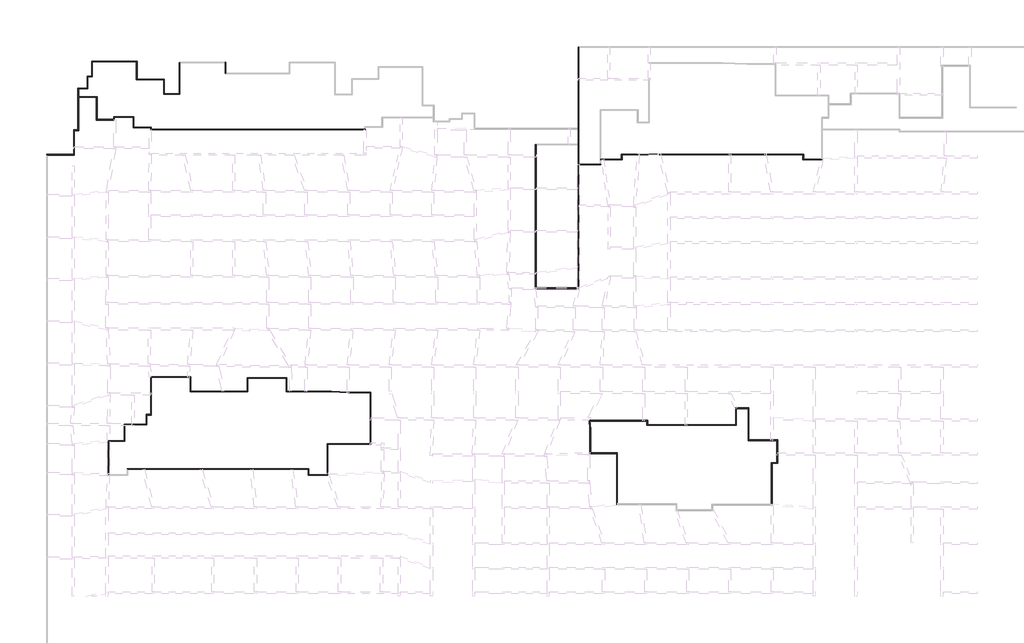
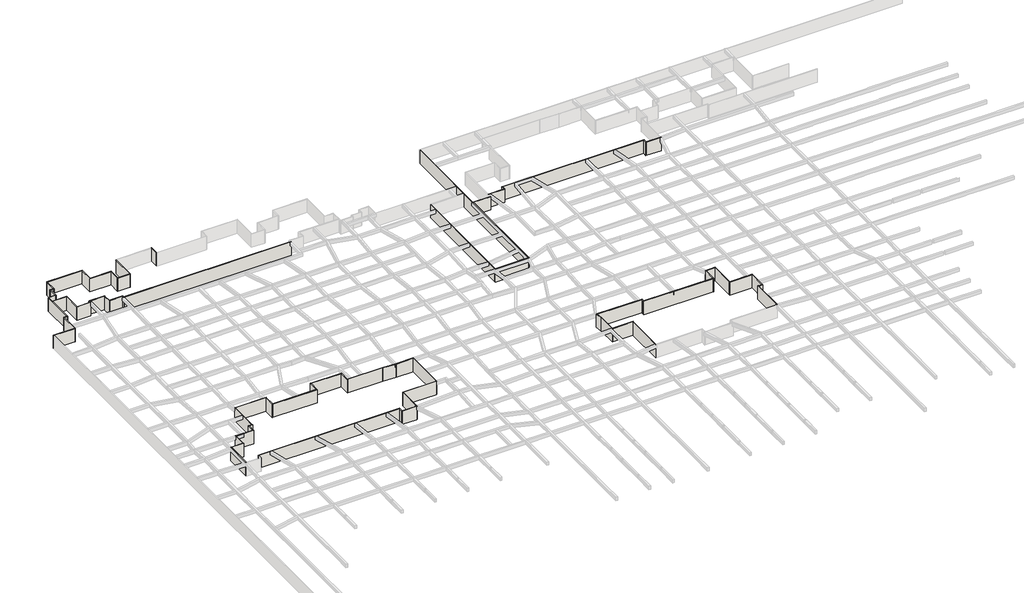
# One storey, part 7 of 45: 69 walls.
"""IFC4 building model written with IfcOpenShell, lengths in millimetres."""

from ifc_helpers import new_model, si_unit, origin, origin_with_axes, place, context, project, spatial, polyline, outline, extrude, faceted_brep, element, save

model = new_model("IFC4")

# Units and contexts
model_context = context("Model", 3, world=origin())
ifc_project = project(units=[si_unit("LENGTHUNIT", "METRE", prefix="MILLI")], contexts=[model_context])

# Site, building, storey
site = spatial("IfcSite", under=ifc_project)
building = spatial("IfcBuilding", under=site)
storey = spatial("IfcBuildingStorey", under=building, Name="户型图", Elevation=0.0)

# Walls
placement = place(None, origin())
element("IfcWall", 1, ObjectType="所有墙体", at=placement, inside=storey, context=model_context, shape_type="Brep", body=[
    faceted_brep([(-138380.5216564, 208531.9876735, 0.0), (-146800.5216564, 208531.9876735, 0.0), (-146800.5216564, 208531.9876735, 3300.0), (-138380.5216564, 208531.9876735, 3300.0), (-138380.5216564, 208411.9876735, 0.0), (-138380.5216564, 208411.9876735, 3300.0), (-138500.5216564, 208411.9876735, 3300.0), (-146680.5216564, 208411.9876735, 3300.0), (-146800.5216564, 208411.9876735, 3300.0), (-146800.5216564, 208411.9876735, 0.0), (-146680.5216564, 208411.9876735, 0.0), (-138500.5216564, 208411.9876735, 0.0)], [[[0, 1, 2, 3]], [[4, 5, 6, 7, 8, 9, 10, 11]], [[1, 0, 4, 11, 10, 9]], [[3, 2, 8, 7, 6, 5]], [[2, 1, 9, 8]], [[0, 3, 5, 4]]]),
])
element("IfcWall", 2, ObjectType="所有墙体", at=placement, inside=storey, context=model_context, shape_type="Brep", body=[
    faceted_brep([(-146800.5216564, 208411.9876735, 0.0), (-146800.5216564, 205731.9876735, 0.0), (-146800.5216564, 205611.9876735, 0.0), (-146800.5216564, 205611.9876735, 3300.0), (-146800.5216564, 205731.9876735, 3300.0), (-146800.5216564, 208411.9876735, 3300.0), (-146680.5216564, 208411.9876735, 0.0), (-146680.5216564, 208411.9876735, 3300.0), (-146680.5216564, 205611.9876735, 3300.0), (-146680.5216564, 205611.9876735, 0.0)], [[[0, 1, 2, 3, 4, 5]], [[6, 7, 8, 9]], [[2, 1, 0, 6, 9]], [[5, 4, 3, 8, 7]], [[0, 5, 7, 6]], [[3, 2, 9, 8]]]),
])
element("IfcWall", 3, ObjectType="所有墙体", at=placement, inside=storey, context=model_context, shape_type="Brep", body=[
    faceted_brep([(-146800.5216564, 205731.9876735, 0.0), (-147600.5216564, 205731.9876735, 0.0), (-147600.5216564, 205731.9876735, 3300.0), (-146800.5216564, 205731.9876735, 3300.0), (-146800.5216564, 205611.9876735, 0.0), (-146800.5216564, 205611.9876735, 3300.0), (-147480.5216564, 205611.9876735, 3300.0), (-147600.5216564, 205611.9876735, 3300.0), (-147600.5216564, 205611.9876735, 0.0), (-147480.5216564, 205611.9876735, 0.0)], [[[0, 1, 2, 3]], [[4, 5, 6, 7, 8, 9]], [[1, 0, 4, 9, 8]], [[3, 2, 7, 6, 5]], [[0, 3, 5, 4]], [[2, 1, 8, 7]]]),
])
element("IfcWall", 4, ObjectType="所有墙体", at=placement, inside=storey, context=model_context, shape_type="Brep", body=[
    faceted_brep([(-147600.5216564, 205611.9876735, 0.0), (-147600.5216564, 203531.9876735, 0.0), (-147600.5216564, 203411.9876735, 0.0), (-147600.5216564, 203411.9876735, 3300.0), (-147600.5216564, 203531.9876735, 3300.0), (-147600.5216564, 205611.9876735, 3300.0), (-147480.5216564, 205611.9876735, 0.0), (-147480.5216564, 205611.9876735, 3300.0), (-147480.5216564, 203411.9876735, 3300.0), (-147480.5216564, 203411.9876735, 0.0)], [[[0, 1, 2, 3, 4, 5]], [[6, 7, 8, 9]], [[2, 1, 0, 6, 9]], [[5, 4, 3, 8, 7]], [[0, 5, 7, 6]], [[3, 2, 9, 8]]]),
])
element("IfcWall", 5, ObjectType="所有墙体", at=placement, inside=storey, context=model_context, shape_type="Brep", body=[
    faceted_brep([(-147600.5216564, 203531.9876735, 0.0), (-149300.5216564, 203531.9876735, 0.0), (-149300.5216564, 203531.9876735, 3300.0), (-147600.5216564, 203531.9876735, 3300.0), (-147600.5216564, 203411.9876735, 0.0), (-147600.5216564, 203411.9876735, 3300.0), (-149180.5216564, 203411.9876735, 3300.0), (-149300.5216564, 203411.9876735, 3300.0), (-149300.5216564, 203411.9876735, 0.0), (-149180.5216564, 203411.9876735, 0.0)], [[[0, 1, 2, 3]], [[4, 5, 6, 7, 8, 9]], [[1, 0, 4, 9, 8]], [[3, 2, 7, 6, 5]], [[0, 3, 5, 4]], [[2, 1, 8, 7]]]),
])
element("IfcWall", 6, ObjectType="所有墙体", at=placement, inside=storey, context=model_context, shape_type="Brep", body=[
    faceted_brep([(-149300.5216564, 203411.9876735, 0.0), (-149300.5216564, 195831.9876735, 0.0), (-149300.5216564, 195711.9876735, 0.0), (-149300.5216564, 195711.9876735, 3300.0), (-149300.5216564, 195831.9876735, 3300.0), (-149300.5216564, 203411.9876735, 3300.0), (-149180.5216564, 203411.9876735, 0.0), (-149180.5216564, 203411.9876735, 3300.0), (-149180.5216564, 201971.9876735, 3300.0), (-149180.5216564, 201851.9876735, 3300.0), (-149180.5216564, 195711.9876735, 3300.0), (-149180.5216564, 195711.9876735, 0.0), (-149180.5216564, 201851.9876735, 0.0), (-149180.5216564, 201971.9876735, 0.0)], [[[0, 1, 2, 3, 4, 5]], [[6, 7, 8, 9, 10, 11, 12, 13]], [[2, 1, 0, 6, 13, 12, 11]], [[5, 4, 3, 10, 9, 8, 7]], [[0, 5, 7, 6]], [[3, 2, 11, 10]]]),
])
element("IfcWall", 7, ObjectType="所有墙体", at=placement, inside=storey, context=model_context, shape_type="Brep", body=[
    faceted_brep([(-149300.5216564, 195831.9876735, 0.0), (-150100.5216564, 195831.9876735, 0.0), (-150100.5216564, 195831.9876735, 3300.0), (-149300.5216564, 195831.9876735, 3300.0), (-149300.5216564, 195711.9876735, 0.0), (-149300.5216564, 195711.9876735, 3300.0), (-149980.5216564, 195711.9876735, 3300.0), (-150100.5216564, 195711.9876735, 3300.0), (-150100.5216564, 195711.9876735, 0.0), (-149980.5216564, 195711.9876735, 0.0)], [[[0, 1, 2, 3]], [[4, 5, 6, 7, 8, 9]], [[1, 0, 4, 9, 8]], [[3, 2, 7, 6, 5]], [[0, 3, 5, 4]], [[2, 1, 8, 7]]]),
])
element("IfcWall", 8, ObjectType="所有墙体", at=placement, inside=storey, context=model_context, shape_type="Brep", body=[
    faceted_brep([(-150100.5216564, 195711.9876735, 0.0), (-150100.5216564, 191331.9876735, 0.0), (-150100.5216564, 191211.9876735, 0.0), (-150100.5216564, 191211.9876735, 3300.0), (-150100.5216564, 191331.9876735, 3300.0), (-150100.5216564, 195711.9876735, 3300.0), (-149980.5216564, 195711.9876735, 0.0), (-149980.5216564, 195711.9876735, 3300.0), (-149980.5216564, 191211.9876735, 3300.0), (-149980.5216564, 191211.9876735, 0.0)], [[[0, 1, 2, 3, 4, 5]], [[6, 7, 8, 9]], [[2, 1, 0, 6, 9]], [[5, 4, 3, 8, 7]], [[0, 5, 7, 6]], [[3, 2, 9, 8]]]),
])
element("IfcWall", 9, ObjectType="所有墙体", at=placement, inside=storey, context=model_context, shape_type="Brep", body=[
    faceted_brep([(-150100.5216564, 191331.9876735, 0.0), (-155100.5216564, 191331.9876735, 0.0), (-155100.5216564, 191331.9876735, 3300.0), (-150100.5216564, 191331.9876735, 3300.0), (-150100.5216564, 191211.9876735, 0.0), (-150100.5216564, 191211.9876735, 3300.0), (-154980.5216564, 191211.9876735, 3300.0), (-155100.5216564, 191211.9876735, 3300.0), (-155100.5216564, 191211.9876735, 0.0), (-154980.5216564, 191211.9876735, 0.0)], [[[0, 1, 2, 3]], [[4, 5, 6, 7, 8, 9]], [[1, 0, 4, 9, 8]], [[3, 2, 7, 6, 5]], [[0, 3, 5, 4]], [[2, 1, 8, 7]]]),
])
element("IfcWall", 10, ObjectType="所有墙体", at=placement, inside=storey, context=model_context, shape_type="Brep", body=[
    faceted_brep([(-121980.5216564, 206331.9876735, 0.0), (-121980.5216564, 208331.9876735, 0.0), (-121980.5216564, 208331.9876735, 3300.0), (-121980.5216564, 206331.9876735, 3300.0), (-122100.5216564, 206331.9876735, 0.0), (-122100.5216564, 206331.9876735, 3300.0), (-122100.5216564, 208211.9876735, 3300.0), (-122100.5216564, 208331.9876735, 3300.0), (-122100.5216564, 208331.9876735, 0.0), (-122100.5216564, 208211.9876735, 0.0)], [[[0, 1, 2, 3]], [[4, 5, 6, 7, 8, 9]], [[1, 0, 4, 9, 8]], [[3, 2, 7, 6, 5]], [[0, 3, 5, 4]], [[2, 1, 8, 7]]]),
])
element("IfcWall", 11, ObjectType="所有墙体", at=placement, inside=storey, context=model_context, shape_type="Brep", body=[
    faceted_brep([(-130600.5216564, 208211.9876735, 0.0), (-130600.5216564, 202531.9876735, 0.0), (-130600.5216564, 202411.9876735, 0.0), (-130600.5216564, 202411.9876735, 3300.0), (-130600.5216564, 202531.9876735, 3300.0), (-130600.5216564, 208211.9876735, 3300.0), (-130480.5216564, 208211.9876735, 0.0), (-130480.5216564, 208211.9876735, 3300.0), (-130480.5216564, 202411.9876735, 3300.0), (-130480.5216564, 202411.9876735, 0.0)], [[[0, 1, 2, 3, 4, 5]], [[6, 7, 8, 9]], [[2, 1, 0, 6, 9]], [[5, 4, 3, 8, 7]], [[0, 5, 7, 6]], [[3, 2, 9, 8]]]),
])
element("IfcWall", 12, ObjectType="所有墙体", at=placement, inside=storey, context=model_context, shape_type="Brep", body=[
    faceted_brep([(-130600.5216564, 202531.9876735, 0.0), (-133380.5216564, 202531.9876735, 0.0), (-133500.5216564, 202531.9876735, 0.0), (-133500.5216564, 202531.9876735, 3300.0), (-133380.5216564, 202531.9876735, 3300.0), (-130600.5216564, 202531.9876735, 3300.0), (-130600.5216564, 202411.9876735, 0.0), (-130600.5216564, 202411.9876735, 3300.0), (-133500.5216564, 202411.9876735, 3300.0), (-133500.5216564, 202411.9876735, 0.0)], [[[0, 1, 2, 3, 4, 5]], [[6, 7, 8, 9]], [[2, 1, 0, 6, 9]], [[5, 4, 3, 8, 7]], [[0, 5, 7, 6]], [[3, 2, 9, 8]]]),
])
element("IfcWall", 13, ObjectType="所有墙体", at=placement, inside=storey, context=model_context, shape_type="Brep", body=[
    faceted_brep([(-133380.5216564, 202531.9876735, 0.0), (-133380.5216564, 205231.9876735, 0.0), (-133380.5216564, 205231.9876735, 3300.0), (-133380.5216564, 202531.9876735, 3300.0), (-133500.5216564, 202531.9876735, 0.0), (-133500.5216564, 202531.9876735, 3300.0), (-133500.5216564, 205111.9876735, 3300.0), (-133500.5216564, 205231.9876735, 3300.0), (-133500.5216564, 205231.9876735, 0.0), (-133500.5216564, 205111.9876735, 0.0)], [[[0, 1, 2, 3]], [[4, 5, 6, 7, 8, 9]], [[1, 0, 4, 9, 8]], [[3, 2, 7, 6, 5]], [[0, 3, 5, 4]], [[2, 1, 8, 7]]]),
])
element("IfcWall", 14, ObjectType="所有墙体", at=placement, inside=storey, context=model_context, shape_type="Brep", body=[
    faceted_brep([(-133500.5216564, 205231.9876735, 0.0), (-138380.5216564, 205231.9876735, 0.0), (-138500.5216564, 205231.9876735, 0.0), (-138500.5216564, 205231.9876735, 3300.0), (-138380.5216564, 205231.9876735, 3300.0), (-133500.5216564, 205231.9876735, 3300.0), (-133500.5216564, 205111.9876735, 0.0), (-133500.5216564, 205111.9876735, 3300.0), (-138500.5216564, 205111.9876735, 3300.0), (-138500.5216564, 205111.9876735, 0.0)], [[[0, 1, 2, 3, 4, 5]], [[6, 7, 8, 9]], [[2, 1, 0, 6, 9]], [[5, 4, 3, 8, 7]], [[0, 5, 7, 6]], [[3, 2, 9, 8]]]),
])
element("IfcWall", 15, ObjectType="所有墙体", at=placement, inside=storey, context=model_context, shape_type="SweptSolid", body=[
    extrude(outline(polyline([(-138380.5216564, 208411.9876735), (-138380.5216564, 205231.9876735), (-138500.5216564, 205231.9876735), (-138500.5216564, 208411.9876735), (-138380.5216564, 208411.9876735)])), origin_with_axes(), (0.0, 0.0, 1.0), 3300.0),
])
element("IfcWall", 16, ObjectType="所有墙体", at=placement, inside=storey, context=model_context, shape_type="Brep", body=[
    faceted_brep([(-149180.5216564, 201851.9876735, 0.0), (-145900.5216564, 201851.9876735, 0.0), (-145780.5216564, 201851.9876735, 0.0), (-145780.5216564, 201851.9876735, 3300.0), (-145900.5216564, 201851.9876735, 3300.0), (-149180.5216564, 201851.9876735, 3300.0), (-149180.5216564, 201971.9876735, 0.0), (-149180.5216564, 201971.9876735, 3300.0), (-145780.5216564, 201971.9876735, 3300.0), (-145780.5216564, 201971.9876735, 0.0)], [[[0, 1, 2, 3, 4, 5]], [[6, 7, 8, 9]], [[2, 1, 0, 6, 9]], [[5, 4, 3, 8, 7]], [[0, 5, 7, 6]], [[3, 2, 9, 8]]]),
])
element("IfcWall", 17, ObjectType="所有墙体", at=placement, inside=storey, context=model_context, shape_type="Brep", body=[
    faceted_brep([(-145900.5216564, 201851.9876735, 0.0), (-145900.5216564, 197651.9876735, 0.0), (-145900.5216564, 197651.9876735, 3300.0), (-145900.5216564, 201851.9876735, 3300.0), (-145780.5216564, 201851.9876735, 0.0), (-145780.5216564, 201851.9876735, 3300.0), (-145780.5216564, 197771.9876735, 3300.0), (-145780.5216564, 197651.9876735, 3300.0), (-145780.5216564, 197651.9876735, 0.0), (-145780.5216564, 197771.9876735, 0.0)], [[[0, 1, 2, 3]], [[4, 5, 6, 7, 8, 9]], [[1, 0, 4, 9, 8]], [[3, 2, 7, 6, 5]], [[0, 3, 5, 4]], [[2, 1, 8, 7]]]),
])
element("IfcWall", 18, ObjectType="所有墙体", at=placement, inside=storey, context=model_context, shape_type="Brep", body=[
    faceted_brep([(-145780.5216564, 197651.9876735, 0.0), (-142580.5216564, 197651.9876735, 0.0), (-142580.5216564, 197651.9876735, 3300.0), (-145780.5216564, 197651.9876735, 3300.0), (-145780.5216564, 197771.9876735, 0.0), (-145780.5216564, 197771.9876735, 3300.0), (-142700.5216564, 197771.9876735, 3300.0), (-142580.5216564, 197771.9876735, 3300.0), (-142580.5216564, 197771.9876735, 0.0), (-142700.5216564, 197771.9876735, 0.0)], [[[0, 1, 2, 3]], [[4, 5, 6, 7, 8, 9]], [[1, 0, 4, 9, 8]], [[3, 2, 7, 6, 5]], [[0, 3, 5, 4]], [[2, 1, 8, 7]]]),
])
element("IfcWall", 19, ObjectType="所有墙体", at=placement, inside=storey, context=model_context, shape_type="Brep", body=[
    faceted_brep([(-142580.5216564, 197771.9876735, 0.0), (-142580.5216564, 198151.9876735, 0.0), (-142580.5216564, 198271.9876735, 0.0), (-142580.5216564, 198271.9876735, 3300.0), (-142580.5216564, 198151.9876735, 3300.0), (-142580.5216564, 197771.9876735, 3300.0), (-142700.5216564, 197771.9876735, 0.0), (-142700.5216564, 197771.9876735, 3300.0), (-142700.5216564, 198271.9876735, 3300.0), (-142700.5216564, 198271.9876735, 0.0)], [[[0, 1, 2, 3, 4, 5]], [[6, 7, 8, 9]], [[2, 1, 0, 6, 9]], [[5, 4, 3, 8, 7]], [[0, 5, 7, 6]], [[3, 2, 9, 8]]]),
])
element("IfcWall", 20, ObjectType="所有墙体", at=placement, inside=storey, context=model_context, shape_type="Brep", body=[
    faceted_brep([(-142580.5216564, 198151.9876735, 0.0), (-139100.5216564, 198151.9876735, 0.0), (-138980.5216564, 198151.9876735, 0.0), (-138980.5216564, 198151.9876735, 3300.0), (-139100.5216564, 198151.9876735, 3300.0), (-142580.5216564, 198151.9876735, 3300.0), (-142580.5216564, 198271.9876735, 0.0), (-142580.5216564, 198271.9876735, 3300.0), (-138980.5216564, 198271.9876735, 3300.0), (-138980.5216564, 198271.9876735, 0.0)], [[[0, 1, 2, 3, 4, 5]], [[6, 7, 8, 9]], [[2, 1, 0, 6, 9]], [[5, 4, 3, 8, 7]], [[0, 5, 7, 6]], [[3, 2, 9, 8]]]),
])
element("IfcWall", 21, ObjectType="所有墙体", at=placement, inside=storey, context=model_context, shape_type="Brep", body=[
    faceted_brep([(-139100.5216564, 198151.9876735, 0.0), (-139100.5216564, 196251.9876735, 0.0), (-139100.5216564, 196251.9876735, 3300.0), (-139100.5216564, 198151.9876735, 3300.0), (-138980.5216564, 198151.9876735, 0.0), (-138980.5216564, 198151.9876735, 3300.0), (-138980.5216564, 196371.9876735, 3300.0), (-138980.5216564, 196251.9876735, 3300.0), (-138980.5216564, 196251.9876735, 0.0), (-138980.5216564, 196371.9876735, 0.0)], [[[0, 1, 2, 3]], [[4, 5, 6, 7, 8, 9]], [[1, 0, 4, 9, 8]], [[3, 2, 7, 6, 5]], [[0, 3, 5, 4]], [[2, 1, 8, 7]]]),
])
element("IfcWall", 22, ObjectType="所有墙体", at=placement, inside=storey, context=model_context, shape_type="Brep", body=[
    faceted_brep([(-138980.5216564, 196251.9876735, 0.0), (-135900.5216564, 196251.9876735, 0.0), (-135780.5216564, 196251.9876735, 0.0), (-135780.5216564, 196251.9876735, 3300.0), (-135900.5216564, 196251.9876735, 3300.0), (-138980.5216564, 196251.9876735, 3300.0), (-138980.5216564, 196371.9876735, 0.0), (-138980.5216564, 196371.9876735, 3300.0), (-135780.5216564, 196371.9876735, 3300.0), (-135780.5216564, 196371.9876735, 0.0)], [[[0, 1, 2, 3, 4, 5]], [[6, 7, 8, 9]], [[2, 1, 0, 6, 9]], [[5, 4, 3, 8, 7]], [[0, 5, 7, 6]], [[3, 2, 9, 8]]]),
])
element("IfcWall", 23, ObjectType="所有墙体", at=placement, inside=storey, context=model_context, shape_type="Brep", body=[
    faceted_brep([(-135900.5216564, 196251.9876735, 0.0), (-135900.5216564, 195851.9876735, 0.0), (-135900.5216564, 195851.9876735, 3300.0), (-135900.5216564, 196251.9876735, 3300.0), (-135780.5216564, 196251.9876735, 0.0), (-135780.5216564, 196251.9876735, 3300.0), (-135780.5216564, 195971.9876735, 3300.0), (-135780.5216564, 195851.9876735, 3300.0), (-135780.5216564, 195851.9876735, 0.0), (-135780.5216564, 195971.9876735, 0.0)], [[[0, 1, 2, 3]], [[4, 5, 6, 7, 8, 9]], [[1, 0, 4, 9, 8]], [[3, 2, 7, 6, 5]], [[0, 3, 5, 4]], [[2, 1, 8, 7]]]),
])
element("IfcWall", 24, ObjectType="所有墙体", at=placement, inside=storey, context=model_context, shape_type="Brep", body=[
    faceted_brep([(-135780.5216564, 195851.9876735, 0.0), (-96280.5216564, 195851.9876735, 0.0), (-96280.5216564, 195851.9876735, 3300.0), (-135780.5216564, 195851.9876735, 3300.0), (-135780.5216564, 195971.9876735, 0.0), (-135780.5216564, 195971.9876735, 3300.0), (-96400.5216564, 195971.9876735, 3300.0), (-96280.5216564, 195971.9876735, 3300.0), (-96280.5216564, 195971.9876735, 0.0), (-96400.5216564, 195971.9876735, 0.0)], [[[0, 1, 2, 3]], [[4, 5, 6, 7, 8, 9]], [[1, 0, 4, 9, 8]], [[3, 2, 7, 6, 5]], [[0, 3, 5, 4]], [[2, 1, 8, 7]]]),
])
element("IfcWall", 25, ObjectType="所有墙体", at=placement, inside=storey, context=model_context, shape_type="Brep", body=[
    faceted_brep([(-57000.5216564, 211111.9876735, 0.0), (-57000.5216564, 196131.9876735, 0.0), (-57000.5216564, 196011.9876735, 0.0), (-57000.5216564, 193202.3986126, 0.0), (-57000.5216564, 193082.3986126, 0.0), (-57000.5216564, 166676.8884871, 0.0), (-57000.5216564, 166556.8884871, 0.0), (-57000.5216564, 166556.8884871, 3300.0), (-57000.5216564, 166676.8884871, 3300.0), (-57000.5216564, 193082.3986126, 3300.0), (-57000.5216564, 193202.3986126, 3300.0), (-57000.5216564, 196011.9876735, 3300.0), (-57000.5216564, 196131.9876735, 3300.0), (-57000.5216564, 211111.9876735, 3300.0), (-56880.5216564, 211111.9876735, 0.0), (-56880.5216564, 211111.9876735, 3300.0), (-56880.5216564, 189542.3986126, 3300.0), (-56880.5216564, 189422.3986126, 3300.0), (-56880.5216564, 166556.8884871, 3300.0), (-56880.5216564, 166556.8884871, 0.0), (-56880.5216564, 189422.3986126, 0.0), (-56880.5216564, 189542.3986126, 0.0)], [[[0, 1, 2, 3, 4, 5, 6, 7, 8, 9, 10, 11, 12, 13]], [[14, 15, 16, 17, 18, 19, 20, 21]], [[6, 5, 4, 3, 2, 1, 0, 14, 21, 20, 19]], [[13, 12, 11, 10, 9, 8, 7, 18, 17, 16, 15]], [[7, 6, 19, 18]], [[0, 13, 15, 14]]]),
])
element("IfcWall", 26, ObjectType="所有墙体", at=placement, inside=storey, context=model_context, shape_type="Brep", body=[
    faceted_brep([(-57000.5216564, 166676.8884871, 0.0), (-64742.224124, 166676.8884871, 0.0), (-64862.224124, 166676.8884871, 0.0), (-64862.224124, 166676.8884871, 3300.0), (-64742.224124, 166676.8884871, 3300.0), (-57000.5216564, 166676.8884871, 3300.0), (-57000.5216564, 166556.8884871, 0.0), (-57000.5216564, 166556.8884871, 3300.0), (-64862.224124, 166556.8884871, 3300.0), (-64862.224124, 166556.8884871, 0.0)], [[[0, 1, 2, 3, 4, 5]], [[6, 7, 8, 9]], [[2, 1, 0, 6, 9]], [[5, 4, 3, 8, 7]], [[0, 5, 7, 6]], [[3, 2, 9, 8]]]),
])
element("IfcWall", 27, ObjectType="所有墙体", at=placement, inside=storey, context=model_context, shape_type="SweptSolid", body=[
    extrude(outline(polyline([(-64742.224124, 193082.3986126), (-64742.224124, 166676.8884871), (-64862.224124, 166676.8884871), (-64862.224124, 193082.3986126), (-64742.224124, 193082.3986126)])), origin_with_axes(), (0.0, 0.0, 1.0), 3300.0),
])
element("IfcWall", 28, ObjectType="所有墙体", at=placement, inside=storey, context=model_context, shape_type="Brep", body=[
    faceted_brep([(-56880.5216564, 189422.3986126, 0.0), (-52780.5216564, 189422.3986126, 0.0), (-52780.5216564, 189422.3986126, 3300.0), (-56880.5216564, 189422.3986126, 3300.0), (-56880.5216564, 189542.3986126, 0.0), (-56880.5216564, 189542.3986126, 3300.0), (-52900.5216564, 189542.3986126, 3300.0), (-52780.5216564, 189542.3986126, 3300.0), (-52780.5216564, 189542.3986126, 0.0), (-52900.5216564, 189542.3986126, 0.0)], [[[0, 1, 2, 3]], [[4, 5, 6, 7, 8, 9]], [[1, 0, 4, 9, 8]], [[3, 2, 7, 6, 5]], [[0, 3, 5, 4]], [[2, 1, 8, 7]]]),
])
element("IfcWall", 29, ObjectType="所有墙体", at=placement, inside=storey, context=model_context, shape_type="Brep", body=[
    faceted_brep([(-52780.5216564, 190322.3986126, 0.0), (-48880.5216564, 190322.3986126, 0.0), (-48880.5216564, 190322.3986126, 3300.0), (-52780.5216564, 190322.3986126, 3300.0), (-52780.5216564, 190442.3986126, 0.0), (-52780.5216564, 190442.3986126, 3300.0), (-49000.5216564, 190442.3986126, 3300.0), (-48880.5216564, 190442.3986126, 3300.0), (-48880.5216564, 190442.3986126, 0.0), (-49000.5216564, 190442.3986126, 0.0)], [[[0, 1, 2, 3]], [[4, 5, 6, 7, 8, 9]], [[1, 0, 4, 9, 8]], [[3, 2, 7, 6, 5]], [[0, 3, 5, 4]], [[2, 1, 8, 7]]]),
])
element("IfcWall", 30, ObjectType="所有墙体", at=placement, inside=storey, context=model_context, shape_type="Brep", body=[
    faceted_brep([(-48880.5216564, 190442.3986126, 0.0), (-48880.5216564, 191222.3986126, 0.0), (-48880.5216564, 191342.3986126, 0.0), (-48880.5216564, 191342.3986126, 3300.0), (-48880.5216564, 191222.3986126, 3300.0), (-48880.5216564, 190442.3986126, 3300.0), (-49000.5216564, 190442.3986126, 0.0), (-49000.5216564, 190442.3986126, 3300.0), (-49000.5216564, 191342.3986126, 3300.0), (-49000.5216564, 191342.3986126, 0.0)], [[[0, 1, 2, 3, 4, 5]], [[6, 7, 8, 9]], [[2, 1, 0, 6, 9]], [[5, 4, 3, 8, 7]], [[0, 5, 7, 6]], [[3, 2, 9, 8]]]),
])
element("IfcWall", 31, ObjectType="所有墙体", at=placement, inside=storey, context=model_context, shape_type="Brep", body=[
    faceted_brep([(-48880.5216564, 191222.3986126, 0.0), (-15500.5216564, 191222.3986126, 0.0), (-15380.5216564, 191222.3986126, 0.0), (-15380.5216564, 191222.3986126, 3300.0), (-15500.5216564, 191222.3986126, 3300.0), (-48880.5216564, 191222.3986126, 3300.0), (-48880.5216564, 191342.3986126, 0.0), (-48880.5216564, 191342.3986126, 3300.0), (-15380.5216564, 191342.3986126, 3300.0), (-15380.5216564, 191342.3986126, 0.0)], [[[0, 1, 2, 3, 4, 5]], [[6, 7, 8, 9]], [[2, 1, 0, 6, 9]], [[5, 4, 3, 8, 7]], [[0, 5, 7, 6]], [[3, 2, 9, 8]]]),
])
element("IfcWall", 32, ObjectType="所有墙体", at=placement, inside=storey, context=model_context, shape_type="Brep", body=[
    faceted_brep([(-15500.5216564, 191222.3986126, 0.0), (-15500.5216564, 190322.3986126, 0.0), (-15500.5216564, 190322.3986126, 3300.0), (-15500.5216564, 191222.3986126, 3300.0), (-15380.5216564, 191222.3986126, 0.0), (-15380.5216564, 191222.3986126, 3300.0), (-15380.5216564, 190442.3986126, 3300.0), (-15380.5216564, 190322.3986126, 3300.0), (-15380.5216564, 190322.3986126, 0.0), (-15380.5216564, 190442.3986126, 0.0)], [[[0, 1, 2, 3]], [[4, 5, 6, 7, 8, 9]], [[1, 0, 4, 9, 8]], [[3, 2, 7, 6, 5]], [[0, 3, 5, 4]], [[2, 1, 8, 7]]]),
])
element("IfcWall", 33, ObjectType="所有墙体", at=placement, inside=storey, context=model_context, shape_type="Brep", body=[
    faceted_brep([(-15380.5216564, 190322.3986126, 0.0), (-11926.7821096, 190322.3986126, 0.0), (-11926.7821096, 190322.3986126, 3300.0), (-15380.5216564, 190322.3986126, 3300.0), (-15380.5216564, 190442.3986126, 0.0), (-15380.5216564, 190442.3986126, 3300.0), (-12046.7821096, 190442.3986126, 3300.0), (-11926.7821096, 190442.3986126, 3300.0), (-11926.7821096, 190442.3986126, 0.0), (-12046.7821096, 190442.3986126, 0.0)], [[[0, 1, 2, 3]], [[4, 5, 6, 7, 8, 9]], [[1, 0, 4, 9, 8]], [[3, 2, 7, 6, 5]], [[0, 3, 5, 4]], [[2, 1, 8, 7]]]),
])
element("IfcWall", 34, ObjectType="所有墙体", at=placement, inside=storey, context=model_context, shape_type="Brep", body=[
    faceted_brep([(-140683.5692432, 141410.7814363, 0.0), (-136572.9151571, 141410.7814363, 0.0), (-136572.9151571, 141410.7814363, 3300.0), (-140683.5692432, 141410.7814363, 3300.0), (-140683.5692432, 141530.7814363, 0.0), (-140683.5692432, 141530.7814363, 3300.0), (-136692.9151571, 141530.7814363, 3300.0), (-136572.9151571, 141530.7814363, 3300.0), (-136572.9151571, 141530.7814363, 0.0), (-136692.9151571, 141530.7814363, 0.0)], [[[0, 1, 2, 3]], [[4, 5, 6, 7, 8, 9]], [[1, 0, 4, 9, 8]], [[3, 2, 7, 6, 5]], [[2, 1, 8, 7]], [[0, 3, 5, 4]]]),
])
element("IfcWall", 35, ObjectType="所有墙体", at=placement, inside=storey, context=model_context, shape_type="Brep", body=[
    faceted_brep([(-136572.9151571, 141530.7814363, 0.0), (-136572.9151571, 143210.7814363, 0.0), (-136572.9151571, 143330.7814363, 0.0), (-136572.9151571, 143330.7814363, 3300.0), (-136572.9151571, 143210.7814363, 3300.0), (-136572.9151571, 141530.7814363, 3300.0), (-136692.9151571, 141530.7814363, 0.0), (-136692.9151571, 141530.7814363, 3300.0), (-136692.9151571, 143330.7814363, 3300.0), (-136692.9151571, 143330.7814363, 0.0)], [[[0, 1, 2, 3, 4, 5]], [[6, 7, 8, 9]], [[2, 1, 0, 6, 9]], [[5, 4, 3, 8, 7]], [[0, 5, 7, 6]], [[3, 2, 9, 8]]]),
])
element("IfcWall", 36, ObjectType="所有墙体", at=placement, inside=storey, context=model_context, shape_type="Brep", body=[
    faceted_brep([(-136572.9151571, 143210.7814363, 0.0), (-135772.9151571, 143210.7814363, 0.0), (-135772.9151571, 143210.7814363, 3300.0), (-136572.9151571, 143210.7814363, 3300.0), (-136572.9151571, 143330.7814363, 0.0), (-136572.9151571, 143330.7814363, 3300.0), (-135892.9151571, 143330.7814363, 3300.0), (-135772.9151571, 143330.7814363, 3300.0), (-135772.9151571, 143330.7814363, 0.0), (-135892.9151571, 143330.7814363, 0.0)], [[[0, 1, 2, 3]], [[4, 5, 6, 7, 8, 9]], [[1, 0, 4, 9, 8]], [[3, 2, 7, 6, 5]], [[0, 3, 5, 4]], [[2, 1, 8, 7]]]),
])
element("IfcWall", 37, ObjectType="所有墙体", at=placement, inside=storey, context=model_context, shape_type="Brep", body=[
    faceted_brep([(-135772.9151571, 143330.7814363, 0.0), (-135772.9151571, 150210.7814363, 0.0), (-135772.9151571, 150330.7814363, 0.0), (-135772.9151571, 150330.7814363, 3300.0), (-135772.9151571, 150210.7814363, 3300.0), (-135772.9151571, 143330.7814363, 3300.0), (-135892.9151571, 143330.7814363, 0.0), (-135892.9151571, 143330.7814363, 3300.0), (-135892.9151571, 150330.7814363, 3300.0), (-135892.9151571, 150330.7814363, 0.0)], [[[0, 1, 2, 3, 4, 5]], [[6, 7, 8, 9]], [[2, 1, 0, 6, 9]], [[5, 4, 3, 8, 7]], [[0, 5, 7, 6]], [[3, 2, 9, 8]]]),
])
element("IfcWall", 38, ObjectType="所有墙体", at=placement, inside=storey, context=model_context, shape_type="Brep", body=[
    faceted_brep([(-135772.9151571, 150210.7814363, 0.0), (-128592.9151571, 150210.7814363, 0.0), (-128472.9151571, 150210.7814363, 0.0), (-128472.9151571, 150210.7814363, 3300.0), (-128592.9151571, 150210.7814363, 3300.0), (-135772.9151571, 150210.7814363, 3300.0), (-135772.9151571, 150330.7814363, 0.0), (-135772.9151571, 150330.7814363, 3300.0), (-128472.9151571, 150330.7814363, 3300.0), (-128472.9151571, 150330.7814363, 0.0)], [[[0, 1, 2, 3, 4, 5]], [[6, 7, 8, 9]], [[2, 1, 0, 6, 9]], [[5, 4, 3, 8, 7]], [[0, 5, 7, 6]], [[3, 2, 9, 8]]]),
])
element("IfcWall", 39, ObjectType="所有墙体", at=placement, inside=storey, context=model_context, shape_type="Brep", body=[
    faceted_brep([(-128592.9151571, 150210.7814363, 0.0), (-128592.9151571, 147510.7814363, 0.0), (-128592.9151571, 147510.7814363, 3300.0), (-128592.9151571, 150210.7814363, 3300.0), (-128472.9151571, 150210.7814363, 0.0), (-128472.9151571, 150210.7814363, 3300.0), (-128472.9151571, 147630.7814363, 3300.0), (-128472.9151571, 147510.7814363, 3300.0), (-128472.9151571, 147510.7814363, 0.0), (-128472.9151571, 147630.7814363, 0.0)], [[[0, 1, 2, 3]], [[4, 5, 6, 7, 8, 9]], [[1, 0, 4, 9, 8]], [[3, 2, 7, 6, 5]], [[0, 3, 5, 4]], [[2, 1, 8, 7]]]),
])
element("IfcWall", 40, ObjectType="所有墙体", at=placement, inside=storey, context=model_context, shape_type="Brep", body=[
    faceted_brep([(-128472.9151571, 147510.7814363, 0.0), (-117972.9151571, 147510.7814363, 0.0), (-117972.9151571, 147510.7814363, 3300.0), (-128472.9151571, 147510.7814363, 3300.0), (-128472.9151571, 147630.7814363, 0.0), (-128472.9151571, 147630.7814363, 3300.0), (-118092.9151571, 147630.7814363, 3300.0), (-117972.9151571, 147630.7814363, 3300.0), (-117972.9151571, 147630.7814363, 0.0), (-118092.9151571, 147630.7814363, 0.0)], [[[0, 1, 2, 3]], [[4, 5, 6, 7, 8, 9]], [[1, 0, 4, 9, 8]], [[3, 2, 7, 6, 5]], [[0, 3, 5, 4]], [[2, 1, 8, 7]]]),
])
element("IfcWall", 41, ObjectType="所有墙体", at=placement, inside=storey, context=model_context, shape_type="Brep", body=[
    faceted_brep([(-117972.9151571, 147630.7814363, 0.0), (-117972.9151571, 150010.7814363, 0.0), (-117972.9151571, 150130.7814363, 0.0), (-117972.9151571, 150130.7814363, 3300.0), (-117972.9151571, 150010.7814363, 3300.0), (-117972.9151571, 147630.7814363, 3300.0), (-118092.9151571, 147630.7814363, 0.0), (-118092.9151571, 147630.7814363, 3300.0), (-118092.9151571, 150130.7814363, 3300.0), (-118092.9151571, 150130.7814363, 0.0)], [[[0, 1, 2, 3, 4, 5]], [[6, 7, 8, 9]], [[2, 1, 0, 6, 9]], [[5, 4, 3, 8, 7]], [[0, 5, 7, 6]], [[3, 2, 9, 8]]]),
])
element("IfcWall", 42, ObjectType="所有墙体", at=placement, inside=storey, context=model_context, shape_type="Brep", body=[
    faceted_brep([(-117972.9151571, 150010.7814363, 0.0), (-110892.9151571, 150010.7814363, 0.0), (-110772.9151571, 150010.7814363, 0.0), (-110772.9151571, 150010.7814363, 3300.0), (-110892.9151571, 150010.7814363, 3300.0), (-117972.9151571, 150010.7814363, 3300.0), (-117972.9151571, 150130.7814363, 0.0), (-117972.9151571, 150130.7814363, 3300.0), (-110772.9151571, 150130.7814363, 3300.0), (-110772.9151571, 150130.7814363, 0.0)], [[[0, 1, 2, 3, 4, 5]], [[6, 7, 8, 9]], [[2, 1, 0, 6, 9]], [[5, 4, 3, 8, 7]], [[0, 5, 7, 6]], [[3, 2, 9, 8]]]),
])
element("IfcWall", 43, ObjectType="所有墙体", at=placement, inside=storey, context=model_context, shape_type="Brep", body=[
    faceted_brep([(-110892.9151571, 150010.7814363, 0.0), (-110892.9151571, 147510.7814363, 0.0), (-110892.9151571, 147510.7814363, 3300.0), (-110892.9151571, 150010.7814363, 3300.0), (-110772.9151571, 150010.7814363, 0.0), (-110772.9151571, 150010.7814363, 3300.0), (-110772.9151571, 147630.7814363, 3300.0), (-110772.9151571, 147510.7814363, 3300.0), (-110772.9151571, 147510.7814363, 0.0), (-110772.9151571, 147630.7814363, 0.0)], [[[0, 1, 2, 3]], [[4, 5, 6, 7, 8, 9]], [[1, 0, 4, 9, 8]], [[3, 2, 7, 6, 5]], [[0, 3, 5, 4]], [[2, 1, 8, 7]]]),
])
element("IfcWall", 44, ObjectType="所有墙体", at=placement, inside=storey, context=model_context, shape_type="SweptSolid", body=[
    extrude(outline(polyline([(-102534.7708159, 147510.7814363), (-110772.9151571, 147510.7814363), (-110772.9151571, 147630.7814363), (-102531.0594982, 147630.7814363), (-102534.7708159, 147510.7814363)])), origin_with_axes(), (0.0, 0.0, 1.0), 3300.0),
])
element("IfcWall", 45, ObjectType="所有墙体", at=placement, inside=storey, context=model_context, shape_type="SweptSolid", body=[
    extrude(outline(polyline([(-99445.424902, 147319.5060773), (-102534.7708159, 147510.7814363), (-102531.0594982, 147630.7814363), (-99441.7135844, 147439.5060773), (-99445.424902, 147319.5060773)])), origin_with_axes(), (0.0, 0.0, 1.0), 3300.0),
])
element("IfcWall", 46, ObjectType="所有墙体", at=placement, inside=storey, context=model_context, shape_type="Brep", body=[
    faceted_brep([(-99445.424902, 147319.5060773, 0.0), (-95403.5692432, 147319.5060773, 0.0), (-95283.5692432, 147319.5060773, 0.0), (-95283.5692432, 147319.5060773, 3300.0), (-95403.5692432, 147319.5060773, 3300.0), (-99445.424902, 147319.5060773, 3300.0), (-99441.7135844, 147439.5060773, 0.0), (-99441.7135844, 147439.5060773, 3300.0), (-95283.5692432, 147439.5060773, 3300.0), (-95283.5692432, 147439.5060773, 0.0)], [[[0, 1, 2, 3, 4, 5]], [[6, 7, 8, 9]], [[2, 1, 0, 6, 9]], [[5, 4, 3, 8, 7]], [[0, 5, 7, 6]], [[3, 2, 9, 8]]]),
])
element("IfcWall", 47, ObjectType="所有墙体", at=placement, inside=storey, context=model_context, shape_type="Brep", body=[
    faceted_brep([(-95403.5692432, 147319.5060773, 0.0), (-95403.5692432, 137939.5060773, 0.0), (-95403.5692432, 137819.5060773, 0.0), (-95403.5692432, 137819.5060773, 3300.0), (-95403.5692432, 137939.5060773, 3300.0), (-95403.5692432, 147319.5060773, 3300.0), (-95283.5692432, 147319.5060773, 0.0), (-95283.5692432, 147319.5060773, 3300.0), (-95283.5692432, 137819.5060773, 3300.0), (-95283.5692432, 137819.5060773, 0.0)], [[[0, 1, 2, 3, 4, 5]], [[6, 7, 8, 9]], [[2, 1, 0, 6, 9]], [[5, 4, 3, 8, 7]], [[0, 5, 7, 6]], [[3, 2, 9, 8]]]),
])
element("IfcWall", 48, ObjectType="所有墙体", at=placement, inside=storey, context=model_context, shape_type="Brep", body=[
    faceted_brep([(-95403.5692432, 137939.5060773, 0.0), (-103303.5692432, 137939.5060773, 0.0), (-103303.5692432, 137939.5060773, 3300.0), (-95403.5692432, 137939.5060773, 3300.0), (-95403.5692432, 137819.5060773, 0.0), (-95403.5692432, 137819.5060773, 3300.0), (-103183.5692432, 137819.5060773, 3300.0), (-103303.5692432, 137819.5060773, 3300.0), (-103303.5692432, 137819.5060773, 0.0), (-103183.5692432, 137819.5060773, 0.0)], [[[0, 1, 2, 3]], [[4, 5, 6, 7, 8, 9]], [[1, 0, 4, 9, 8]], [[3, 2, 7, 6, 5]], [[0, 3, 5, 4]], [[2, 1, 8, 7]]]),
])
element("IfcWall", 49, ObjectType="所有墙体", at=placement, inside=storey, context=model_context, shape_type="Brep", body=[
    faceted_brep([(-103303.5692432, 137819.5060773, 0.0), (-103303.5692432, 132195.8564831, 0.0), (-103303.5692432, 132075.8564831, 0.0), (-103303.5692432, 132075.8564831, 3300.0), (-103303.5692432, 132195.8564831, 3300.0), (-103303.5692432, 137819.5060773, 3300.0), (-103183.5692432, 137819.5060773, 0.0), (-103183.5692432, 137819.5060773, 3300.0), (-103183.5692432, 132075.8564831, 3300.0), (-103183.5692432, 132075.8564831, 0.0)], [[[0, 1, 2, 3, 4, 5]], [[6, 7, 8, 9]], [[2, 1, 0, 6, 9]], [[5, 4, 3, 8, 7]], [[0, 5, 7, 6]], [[3, 2, 9, 8]]]),
])
element("IfcWall", 50, ObjectType="所有墙体", at=placement, inside=storey, context=model_context, shape_type="Brep", body=[
    faceted_brep([(-103303.5692432, 132195.8564831, 0.0), (-106683.5692432, 132195.8564831, 0.0), (-106803.5692432, 132195.8564831, 0.0), (-106803.5692432, 132195.8564831, 3300.0), (-106683.5692432, 132195.8564831, 3300.0), (-103303.5692432, 132195.8564831, 3300.0), (-103303.5692432, 132075.8564831, 0.0), (-103303.5692432, 132075.8564831, 3300.0), (-106803.5692432, 132075.8564831, 3300.0), (-106803.5692432, 132075.8564831, 0.0)], [[[0, 1, 2, 3, 4, 5]], [[6, 7, 8, 9]], [[2, 1, 0, 6, 9]], [[5, 4, 3, 8, 7]], [[0, 5, 7, 6]], [[3, 2, 9, 8]]]),
])
element("IfcWall", 51, ObjectType="所有墙体", at=placement, inside=storey, context=model_context, shape_type="Brep", body=[
    faceted_brep([(-106683.5692432, 132195.8564831, 0.0), (-106683.5692432, 133295.8564831, 0.0), (-106683.5692432, 133295.8564831, 3300.0), (-106683.5692432, 132195.8564831, 3300.0), (-106803.5692432, 132195.8564831, 0.0), (-106803.5692432, 132195.8564831, 3300.0), (-106803.5692432, 133175.8564831, 3300.0), (-106803.5692432, 133295.8564831, 3300.0), (-106803.5692432, 133295.8564831, 0.0), (-106803.5692432, 133175.8564831, 0.0)], [[[0, 1, 2, 3]], [[4, 5, 6, 7, 8, 9]], [[1, 0, 4, 9, 8]], [[3, 2, 7, 6, 5]], [[0, 3, 5, 4]], [[2, 1, 8, 7]]]),
])
element("IfcWall", 52, ObjectType="所有墙体", at=placement, inside=storey, context=model_context, shape_type="Brep", body=[
    faceted_brep([(-106803.5692432, 133295.8564831, 0.0), (-140203.5692432, 133295.8564831, 0.0), (-140203.5692432, 133295.8564831, 3300.0), (-106803.5692432, 133295.8564831, 3300.0), (-106803.5692432, 133175.8564831, 0.0), (-106803.5692432, 133175.8564831, 3300.0), (-140083.5692432, 133175.8564831, 3300.0), (-140203.5692432, 133175.8564831, 3300.0), (-140203.5692432, 133175.8564831, 0.0), (-140083.5692432, 133175.8564831, 0.0)], [[[0, 1, 2, 3]], [[4, 5, 6, 7, 8, 9]], [[1, 0, 4, 9, 8]], [[3, 2, 7, 6, 5]], [[0, 3, 5, 4]], [[2, 1, 8, 7]]]),
])
element("IfcWall", 53, ObjectType="所有墙体", at=placement, inside=storey, context=model_context, shape_type="Brep", body=[
    faceted_brep([(-143583.5692432, 132195.8564831, 0.0), (-143583.5692432, 138375.8564831, 0.0), (-143583.5692432, 138495.8564831, 0.0), (-143583.5692432, 138495.8564831, 3300.0), (-143583.5692432, 138375.8564831, 3300.0), (-143583.5692432, 132195.8564831, 3300.0), (-143703.5692432, 132195.8564831, 0.0), (-143703.5692432, 132195.8564831, 3300.0), (-143703.5692432, 138495.8564831, 3300.0), (-143703.5692432, 138495.8564831, 0.0)], [[[0, 1, 2, 3, 4, 5]], [[6, 7, 8, 9]], [[2, 1, 0, 6, 9]], [[5, 4, 3, 8, 7]], [[0, 5, 7, 6]], [[3, 2, 9, 8]]]),
])
element("IfcWall", 54, ObjectType="所有墙体", at=placement, inside=storey, context=model_context, shape_type="Brep", body=[
    faceted_brep([(-143583.5692432, 138375.8564831, 0.0), (-140683.5692432, 138375.8564831, 0.0), (-140683.5692432, 138375.8564831, 3300.0), (-143583.5692432, 138375.8564831, 3300.0), (-143583.5692432, 138495.8564831, 0.0), (-143583.5692432, 138495.8564831, 3300.0), (-140803.5692432, 138495.8564831, 3300.0), (-140683.5692432, 138495.8564831, 3300.0), (-140683.5692432, 138495.8564831, 0.0), (-140803.5692432, 138495.8564831, 0.0)], [[[0, 1, 2, 3]], [[4, 5, 6, 7, 8, 9]], [[1, 0, 4, 9, 8]], [[3, 2, 7, 6, 5]], [[0, 3, 5, 4]], [[2, 1, 8, 7]]]),
])
element("IfcWall", 55, ObjectType="所有墙体", at=placement, inside=storey, context=model_context, shape_type="Brep", body=[
    faceted_brep([(-140683.5692432, 138495.8564831, 0.0), (-140683.5692432, 141410.7814363, 0.0), (-140683.5692432, 141530.7814363, 0.0), (-140683.5692432, 141530.7814363, 3300.0), (-140683.5692432, 141410.7814363, 3300.0), (-140683.5692432, 138495.8564831, 3300.0), (-140803.5692432, 138495.8564831, 0.0), (-140803.5692432, 138495.8564831, 3300.0), (-140803.5692432, 141530.7814363, 3300.0), (-140803.5692432, 141530.7814363, 0.0)], [[[0, 1, 2, 3, 4, 5]], [[6, 7, 8, 9]], [[2, 1, 0, 6, 9]], [[5, 4, 3, 8, 7]], [[0, 5, 7, 6]], [[3, 2, 9, 8]]]),
])
element("IfcWall", 56, ObjectType="所有墙体", at=placement, inside=storey, context=model_context, shape_type="Brep", body=[
    faceted_brep([(-54982.3711745, 142222.9605472, 0.0), (-54807.1090692, 140555.4530019, 0.0), (-54807.1090692, 140555.4530019, 3300.0), (-54982.3711745, 142222.9605472, 3300.0), (-54861.7101809, 142222.9605472, 0.0), (-54861.7101809, 142222.9605472, 3300.0), (-54849.0976727, 142102.9605472, 3300.0), (-54687.1090692, 140561.7419354, 3300.0), (-54687.1090692, 140561.7419354, 0.0), (-54849.0976727, 142102.9605472, 0.0)], [[[0, 1, 2, 3]], [[4, 5, 6, 7, 8, 9]], [[1, 0, 4, 9, 8]], [[3, 2, 7, 6, 5]], [[2, 1, 8, 7]], [[0, 3, 5, 4]]]),
])
element("IfcWall", 57, ObjectType="所有墙体", at=placement, inside=storey, context=model_context, shape_type="Brep", body=[
    faceted_brep([(-54807.1090692, 140555.4530019, 0.0), (-54807.1090692, 136098.5974686, 0.0), (-54807.1090692, 136098.5974686, 3300.0), (-54807.1090692, 140555.4530019, 3300.0), (-54687.1090692, 140561.7419354, 0.0), (-54687.1090692, 140561.7419354, 3300.0), (-54687.1090692, 136218.5974686, 3300.0), (-54687.1090692, 136098.5974686, 3300.0), (-54687.1090692, 136098.5974686, 0.0), (-54687.1090692, 136218.5974686, 0.0)], [[[0, 1, 2, 3]], [[4, 5, 6, 7, 8, 9]], [[1, 0, 4, 9, 8]], [[3, 2, 7, 6, 5]], [[0, 3, 5, 4]], [[2, 1, 8, 7]]]),
])
element("IfcWall", 58, ObjectType="所有墙体", at=placement, inside=storey, context=model_context, shape_type="Brep", body=[
    faceted_brep([(-54687.1090692, 136098.5974686, 0.0), (-49907.1090692, 136098.5974686, 0.0), (-49787.1090692, 136098.5974686, 0.0), (-49787.1090692, 136098.5974686, 3300.0), (-49907.1090692, 136098.5974686, 3300.0), (-54687.1090692, 136098.5974686, 3300.0), (-54687.1090692, 136218.5974686, 0.0), (-54687.1090692, 136218.5974686, 3300.0), (-49787.1090692, 136218.5974686, 3300.0), (-49787.1090692, 136218.5974686, 0.0)], [[[0, 1, 2, 3, 4, 5]], [[6, 7, 8, 9]], [[2, 1, 0, 6, 9]], [[5, 4, 3, 8, 7]], [[0, 5, 7, 6]], [[3, 2, 9, 8]]]),
])
element("IfcWall", 59, ObjectType="所有墙体", at=placement, inside=storey, context=model_context, shape_type="Brep", body=[
    faceted_brep([(-49907.1090692, 136098.5974686, 0.0), (-49907.1090692, 126702.9605472, 0.0), (-49907.1090692, 126702.9605472, 3300.0), (-49907.1090692, 136098.5974686, 3300.0), (-49787.1090692, 136098.5974686, 0.0), (-49787.1090692, 136098.5974686, 3300.0), (-49787.1090692, 126822.9605472, 3300.0), (-49787.1090692, 126702.9605472, 3300.0), (-49787.1090692, 126702.9605472, 0.0), (-49787.1090692, 126822.9605472, 0.0)], [[[0, 1, 2, 3]], [[4, 5, 6, 7, 8, 9]], [[1, 0, 4, 9, 8]], [[3, 2, 7, 6, 5]], [[0, 3, 5, 4]], [[2, 1, 8, 7]]]),
])
element("IfcWall", 60, ObjectType="所有墙体", at=placement, inside=storey, context=model_context, shape_type="Brep", body=[
    faceted_brep([(-21187.1090692, 126722.9605472, 0.0), (-21187.1090692, 134302.9605472, 0.0), (-21187.1090692, 134422.9605472, 0.0), (-21187.1090692, 134422.9605472, 3300.0), (-21187.1090692, 134302.9605472, 3300.0), (-21187.1090692, 126722.9605472, 3300.0), (-21307.1090692, 126722.9605472, 0.0), (-21307.1090692, 126722.9605472, 3300.0), (-21307.1090692, 134422.9605472, 3300.0), (-21307.1090692, 134422.9605472, 0.0)], [[[0, 1, 2, 3, 4, 5]], [[6, 7, 8, 9]], [[2, 1, 0, 6, 9]], [[5, 4, 3, 8, 7]], [[0, 5, 7, 6]], [[3, 2, 9, 8]]]),
])
element("IfcWall", 61, ObjectType="所有墙体", at=placement, inside=storey, context=model_context, shape_type="Brep", body=[
    faceted_brep([(-21187.1090692, 134302.9605472, 0.0), (-20187.1090692, 134302.9605472, 0.0), (-20187.1090692, 134302.9605472, 3300.0), (-21187.1090692, 134302.9605472, 3300.0), (-21187.1090692, 134422.9605472, 0.0), (-21187.1090692, 134422.9605472, 3300.0), (-20307.1090692, 134422.9605472, 3300.0), (-20187.1090692, 134422.9605472, 3300.0), (-20187.1090692, 134422.9605472, 0.0), (-20307.1090692, 134422.9605472, 0.0)], [[[0, 1, 2, 3]], [[4, 5, 6, 7, 8, 9]], [[1, 0, 4, 9, 8]], [[3, 2, 7, 6, 5]], [[0, 3, 5, 4]], [[2, 1, 8, 7]]]),
])
element("IfcWall", 62, ObjectType="所有墙体", at=placement, inside=storey, context=model_context, shape_type="Brep", body=[
    faceted_brep([(-20187.1090692, 134422.9605472, 0.0), (-20187.1090692, 138622.9605472, 0.0), (-20187.1090692, 138622.9605472, 3300.0), (-20187.1090692, 134422.9605472, 3300.0), (-20307.1090692, 134422.9605472, 0.0), (-20307.1090692, 134422.9605472, 3300.0), (-20307.1090692, 138502.9605472, 3300.0), (-20307.1090692, 138622.9605472, 3300.0), (-20307.1090692, 138622.9605472, 0.0), (-20307.1090692, 138502.9605472, 0.0)], [[[0, 1, 2, 3]], [[4, 5, 6, 7, 8, 9]], [[1, 0, 4, 9, 8]], [[3, 2, 7, 6, 5]], [[0, 3, 5, 4]], [[2, 1, 8, 7]]]),
])
element("IfcWall", 63, ObjectType="所有墙体", at=placement, inside=storey, context=model_context, shape_type="Brep", body=[
    faceted_brep([(-20307.1090692, 138622.9605472, 0.0), (-25487.1090692, 138622.9605472, 0.0), (-25607.1090692, 138622.9605472, 0.0), (-25607.1090692, 138622.9605472, 3300.0), (-25487.1090692, 138622.9605472, 3300.0), (-20307.1090692, 138622.9605472, 3300.0), (-20307.1090692, 138502.9605472, 0.0), (-20307.1090692, 138502.9605472, 3300.0), (-25607.1090692, 138502.9605472, 3300.0), (-25607.1090692, 138502.9605472, 0.0)], [[[0, 1, 2, 3, 4, 5]], [[6, 7, 8, 9]], [[2, 1, 0, 6, 9]], [[5, 4, 3, 8, 7]], [[0, 5, 7, 6]], [[3, 2, 9, 8]]]),
])
element("IfcWall", 64, ObjectType="所有墙体", at=placement, inside=storey, context=model_context, shape_type="Brep", body=[
    faceted_brep([(-25487.1090692, 138622.9605472, 0.0), (-25487.1090692, 144522.9605472, 0.0), (-25487.1090692, 144522.9605472, 3300.0), (-25487.1090692, 138622.9605472, 3300.0), (-25607.1090692, 138622.9605472, 0.0), (-25607.1090692, 138622.9605472, 3300.0), (-25607.1090692, 144402.9605472, 3300.0), (-25607.1090692, 144522.9605472, 3300.0), (-25607.1090692, 144522.9605472, 0.0), (-25607.1090692, 144402.9605472, 0.0)], [[[0, 1, 2, 3]], [[4, 5, 6, 7, 8, 9]], [[1, 0, 4, 9, 8]], [[3, 2, 7, 6, 5]], [[0, 3, 5, 4]], [[2, 1, 8, 7]]]),
])
element("IfcWall", 65, ObjectType="所有墙体", at=placement, inside=storey, context=model_context, shape_type="Brep", body=[
    faceted_brep([(-25607.1090692, 144522.9605472, 0.0), (-27907.1090692, 144522.9605472, 0.0), (-27907.1090692, 144522.9605472, 3300.0), (-25607.1090692, 144522.9605472, 3300.0), (-25607.1090692, 144402.9605472, 0.0), (-25607.1090692, 144402.9605472, 3300.0), (-27787.1090692, 144402.9605472, 3300.0), (-27907.1090692, 144402.9605472, 3300.0), (-27907.1090692, 144402.9605472, 0.0), (-27787.1090692, 144402.9605472, 0.0)], [[[0, 1, 2, 3]], [[4, 5, 6, 7, 8, 9]], [[1, 0, 4, 9, 8]], [[3, 2, 7, 6, 5]], [[0, 3, 5, 4]], [[2, 1, 8, 7]]]),
])
element("IfcWall", 66, ObjectType="所有墙体", at=placement, inside=storey, context=model_context, shape_type="Brep", body=[
    faceted_brep([(-27907.1090692, 144402.9605472, 0.0), (-27907.1090692, 141422.9605472, 0.0), (-27907.1090692, 141302.9605472, 0.0), (-27907.1090692, 141302.9605472, 3300.0), (-27907.1090692, 141422.9605472, 3300.0), (-27907.1090692, 144402.9605472, 3300.0), (-27787.1090692, 144402.9605472, 0.0), (-27787.1090692, 144402.9605472, 3300.0), (-27787.1090692, 141302.9605472, 3300.0), (-27787.1090692, 141302.9605472, 0.0)], [[[0, 1, 2, 3, 4, 5]], [[6, 7, 8, 9]], [[2, 1, 0, 6, 9]], [[5, 4, 3, 8, 7]], [[0, 5, 7, 6]], [[3, 2, 9, 8]]]),
])
element("IfcWall", 67, ObjectType="所有墙体", at=placement, inside=storey, context=model_context, shape_type="Brep", body=[
    faceted_brep([(-27907.1090692, 141422.9605472, 0.0), (-44187.1090692, 141422.9605472, 0.0), (-44307.1090692, 141422.9605472, 0.0), (-44307.1090692, 141422.9605472, 3300.0), (-44187.1090692, 141422.9605472, 3300.0), (-27907.1090692, 141422.9605472, 3300.0), (-27907.1090692, 141302.9605472, 0.0), (-27907.1090692, 141302.9605472, 3300.0), (-44307.1090692, 141302.9605472, 3300.0), (-44307.1090692, 141302.9605472, 0.0)], [[[0, 1, 2, 3, 4, 5]], [[6, 7, 8, 9]], [[2, 1, 0, 6, 9]], [[5, 4, 3, 8, 7]], [[0, 5, 7, 6]], [[3, 2, 9, 8]]]),
])
element("IfcWall", 68, ObjectType="所有墙体", at=placement, inside=storey, context=model_context, shape_type="Brep", body=[
    faceted_brep([(-44187.1090692, 141422.9605472, 0.0), (-44187.1090692, 142222.9605472, 0.0), (-44187.1090692, 142222.9605472, 3300.0), (-44187.1090692, 141422.9605472, 3300.0), (-44307.1090692, 141422.9605472, 0.0), (-44307.1090692, 141422.9605472, 3300.0), (-44307.1090692, 142102.9605472, 3300.0), (-44307.1090692, 142222.9605472, 3300.0), (-44307.1090692, 142222.9605472, 0.0), (-44307.1090692, 142102.9605472, 0.0)], [[[0, 1, 2, 3]], [[4, 5, 6, 7, 8, 9]], [[1, 0, 4, 9, 8]], [[3, 2, 7, 6, 5]], [[0, 3, 5, 4]], [[2, 1, 8, 7]]]),
])
element("IfcWall", 69, ObjectType="所有墙体", at=placement, inside=storey, context=model_context, shape_type="SweptSolid", body=[
    extrude(outline(polyline([(-54861.7101809, 142222.9605472), (-44307.1090692, 142222.9605472), (-44307.1090692, 142102.9605472), (-54849.0976727, 142102.9605472), (-54861.7101809, 142222.9605472)])), origin_with_axes(), (0.0, 0.0, 1.0), 3300.0),
])

save(model, "model.ifc")

# Revit data of these elements
# Type "所有墙体"
#   Layers, outside or top first: 120 mm "默认" (function 1)
# Elements 1, 2, 3, 4, 5, 6, 7, 8, 9, 10, 11, 12, 13, 14, 15, 16, 17, 18, 19, 20, 21, 22, 23, 24, 25, 26, 27, 28, 29, 30, 31, 32, 33, 34, 35, 36, 37, 38, 39, 40, 41, 42, 43, 44, 45, 46, 47, 48, 49, 50, 51, 52, 53, 54, 55, 56, 57, 58, 59, 60, 61, 62, 63, 64, 65, 66, 67, 68, 69 (IfcWall, "所有墙体")
#   Top Offset = 0 mm
#   Base Offset = 0 mm
#   wall height = 3300 mm
#   Phase Created = 新构造
#   Base Constraint = 户型图
#   Top Constraint = 层高
#   Materials on its faces: "默认"
# Materials
#   "默认": class "其他", colour RGB 192 192 192, transparency 0, Cost = 0
